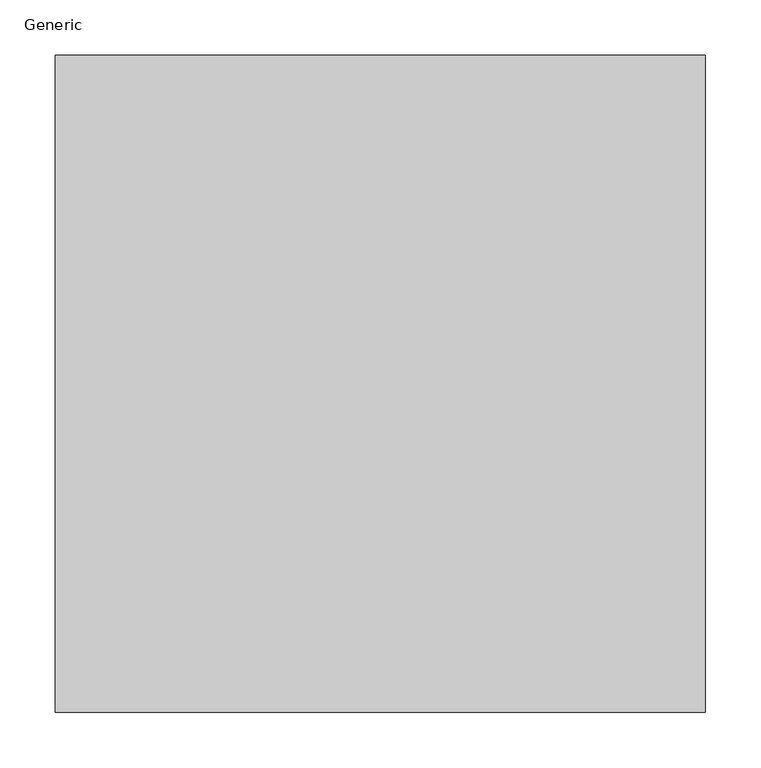
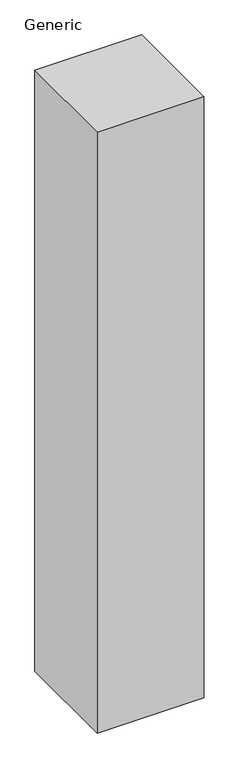
"""IFC4 building model written with IfcOpenShell, lengths in millimetres: column geometry, WWm-ConcreteRectangular-Instance : Generic."""

from ifc_helpers import new_model, si_unit, frame, origin, place, context, project, spatial, polyline, outline, extrude, source, transform, mapped, element, save


def generic_3073c1fe(model_context):
    return source(origin(), model_context, "Body", "SweptSolid", [
        extrude(outline(polyline([(283.4553773, 289.5868214), (283.4553773, -304.8), (-304.8, -304.8), (-304.8, 289.5868214), (283.4553773, 289.5868214)])), frame((0.0, 0.0, 14000.0), z_axis=(0.0, 0.0, 1.0), x_axis=(1.0, 0.0, 0.0)), (0.0, 0.0, 1.0), 3500.0),
    ])


if __name__ == "__main__":
    model = new_model("IFC4")
    model_context = context("Model", 3, world=origin())
    ifc_project = project(units=[si_unit("LENGTHUNIT", "METRE", prefix="MILLI")], contexts=[model_context])
    site = spatial("IfcSite", under=ifc_project)
    building = spatial("IfcBuilding", under=site)
    placement = place(None, origin())
    generic_shape = generic_3073c1fe(model_context)
    element("IfcColumn", 1, ObjectType="WWm-ConcreteRectangular-Instance : Generic", at=placement, inside=building, context=model_context, shape_type="MappedRepresentation", body=[
        mapped(generic_shape, transform((0.0, 0.0, 0.0), x_axis=(1.0, 0.0, 0.0), y_axis=(0.0, 1.0, 0.0), z_axis=(0.0, 0.0, 1.0))),
    ])
    save(model, "model.ifc")

# Revit data of these elements
# Type "WWm-ConcreteRectangular-Instance : Generic"
#   Depth [instance default] = 600 mm
#   Offset Base = 0 mm
#   Offset Top = 0 mm
#   Width [instance default] = 600 mm
#   Material = WW-EC-CR-CastInPlace
#   Assembly Code = ""
# Element 1 (IfcColumn, "WWm-ConcreteRectangular-Instance : Generic")
#   Depth = 594.387 mm
#   Width = 588.255 mm
#   Materials on its faces: "WW-EC-CR-CastInPlace"
# Materials
#   "WW-EC-CR-CastInPlace": class "Concrete", colour RGB 255 255 255, transparency 0, Comments = "If region requests all-white model, remove image from asset", Description = "Cast in Place Concrete", Cost = 0
